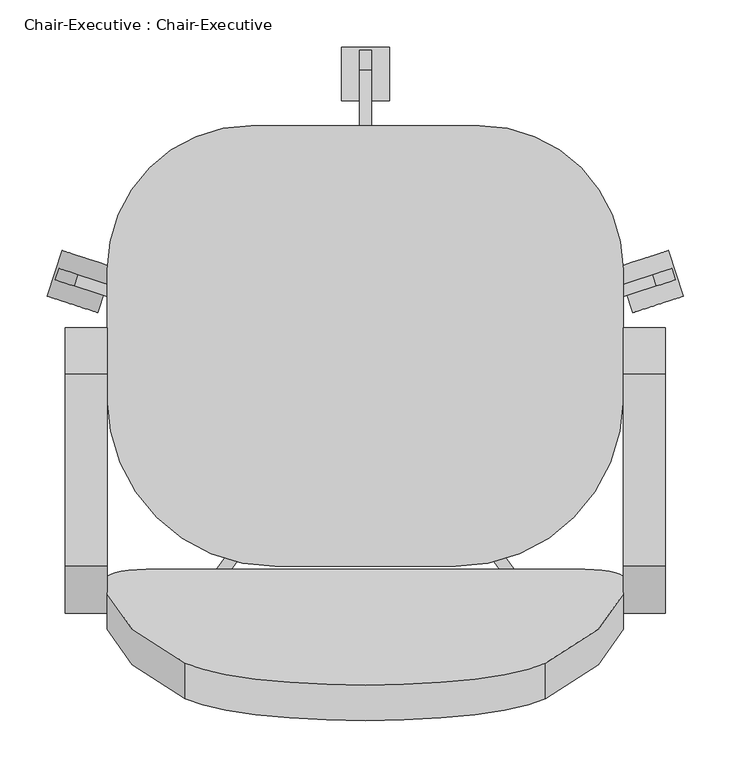
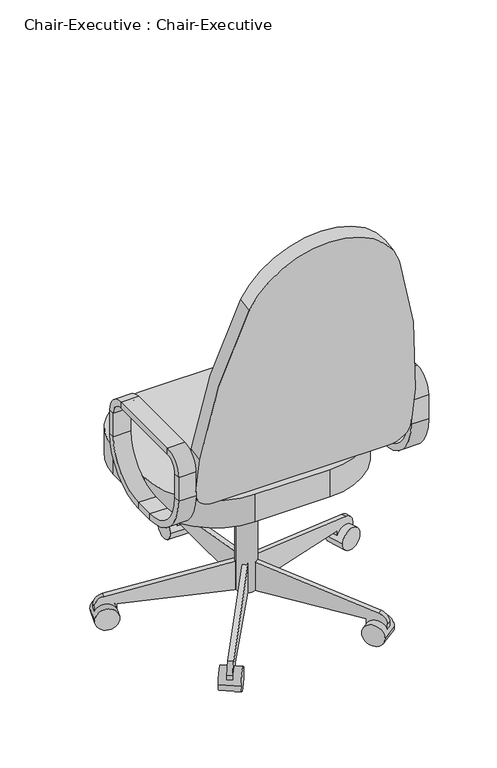
"""IFC4 building model written with IfcOpenShell, lengths in millimetres: furniture geometry, Chair-Executive : Chair-Executive."""

import ifcopenshell
import ifcopenshell.guid

model = None  # the IFC model being written
_history = None  # IfcOwnerHistory: only IFC2X3 demands one
_inside = {}  # id of a spatial element -> (the spatial element, [elements in it])
_under = {}  # id of a project, library or spatial element -> (it, [spatial elements below it])
_declared = {}  # id of a project -> (the project, [libraries it declares])
_typed = {}  # id of a type object -> (the type object, [elements of that type])
_made_of = {}  # id of a material, layer set ... -> (it, [elements and type objects made of it])


def new_model(schema):
    """Start an empty IFC model of exactly this schema.

    Asked for "IFC4X3", IfcOpenShell would pick the latest addendum, in which some entities
    have other attributes; the version numbers below select the first issue.
    IFC2X3 requires an IfcOwnerHistory on every rooted entity: one is made here for all.
    """
    global model, _history
    if schema == "IFC4X3":
        model = ifcopenshell.file(schema_version=(4, 3, 0, 0))
    else:
        model = ifcopenshell.file(schema=schema)
    _inside.clear()
    _under.clear()
    _declared.clear()
    _typed.clear()
    _made_of.clear()
    _history = None
    if model.schema == "IFC2X3":
        org = make("IfcOrganization", Name="unknown")
        user = make(
            "IfcPersonAndOrganization",
            ThePerson=make("IfcPerson", FamilyName="unknown"),
            TheOrganization=org,
        )
        app = make(
            "IfcApplication",
            ApplicationDeveloper=org,
            Version="unknown",
            ApplicationFullName="unknown",
            ApplicationIdentifier="unknown",
        )
        _history = make(
            "IfcOwnerHistory",
            OwningUser=user,
            OwningApplication=app,
            ChangeAction="ADDED",
            CreationDate=0,
        )
    return model


def make(cls, **values):
    """One entity of the class cls with the attributes given. An attribute that is None is left unset."""
    return model.create_entity(
        cls, **{name: value for name, value in values.items() if value is not None}
    )


def rooted(cls, **values):
    """An entity with a GlobalId (a new one), such as an element, a storey or a relation."""
    return make(cls, GlobalId=ifcopenshell.guid.new(), OwnerHistory=_history, **values)


def si_unit(unit_type, name, prefix=None):
    """IfcSIUnit, for example si_unit("LENGTHUNIT", "METRE", prefix="MILLI")."""
    return make("IfcSIUnit", UnitType=unit_type, Prefix=prefix, Name=name)


def assignment(units):
    """IfcUnitAssignment: the units of a project."""
    return None if units is None else make("IfcUnitAssignment", Units=units)


def point(xyz):
    """IfcCartesianPoint."""
    return None if xyz is None else make("IfcCartesianPoint", Coordinates=xyz)


def direction(xyz):
    """IfcDirection."""
    return None if xyz is None else make("IfcDirection", DirectionRatios=xyz)


def frame(location, z_axis=None, x_axis=None):
    """IfcAxis2Placement3D, a coordinate frame: its origin and axes. An axis left out is left unset."""
    return make(
        "IfcAxis2Placement3D",
        Location=point(location),
        Axis=direction(z_axis),
        RefDirection=direction(x_axis),
    )


def frame_2d(location, x_axis=None):
    """IfcAxis2Placement2D, a coordinate frame in the plane: its origin and x axis."""
    return make(
        "IfcAxis2Placement2D", Location=point(location), RefDirection=direction(x_axis)
    )


def origin():
    """The frame at (0, 0, 0) with its axes left unset."""
    return frame((0.0, 0.0, 0.0))


def place(relative_to, where):
    """IfcLocalPlacement: puts the frame where relative to a parent placement (None: the world)."""
    return make(
        "IfcLocalPlacement", PlacementRelTo=relative_to, RelativePlacement=where
    )


def context(
    kind, dimensions, precision=None, world=None, true_north=None, identifier=None
):
    """IfcGeometricRepresentationContext, for example the 3D "Model" context."""
    return make(
        "IfcGeometricRepresentationContext",
        ContextIdentifier=identifier,
        ContextType=kind,
        CoordinateSpaceDimension=dimensions,
        Precision=precision,
        WorldCoordinateSystem=world,
        TrueNorth=true_north,
    )


def project(units=None, contexts=None):
    """IfcProject with its units and contexts."""
    return rooted(
        "IfcProject",
        Name="project",
        RepresentationContexts=contexts,
        UnitsInContext=assignment(units),
    )


def spatial(cls, under=None, at=None, **own):
    """A site, building, storey or space (cls), placed at a placement, below another one or the project."""
    s = rooted(cls, ObjectPlacement=at, **own)
    if under is not None:
        _under.setdefault(under.id(), (under, []))[1].append(s)
    return s


def polyline(points):
    """IfcPolyline through the points."""
    return make("IfcPolyline", Points=[point(p) for p in points])


def circle_curve(where, radius):
    """IfcCircle in the frame where."""
    return make("IfcCircle", Position=where, Radius=radius)


def trimmed(basis, trim1, trim2, sense, master):
    """IfcTrimmedCurve: the piece of a basis curve between two trims."""
    return make(
        "IfcTrimmedCurve",
        BasisCurve=basis,
        Trim1=trim1,
        Trim2=trim2,
        SenseAgreement=sense,
        MasterRepresentation=master,
    )


def segment(curve, same_sense, transition):
    """IfcCompositeCurveSegment."""
    return make(
        "IfcCompositeCurveSegment",
        Transition=transition,
        SameSense=same_sense,
        ParentCurve=curve,
    )


def composite_curve(segments, self_intersect=None):
    """IfcCompositeCurve: segments joined end to end."""
    return make("IfcCompositeCurve", Segments=segments, SelfIntersect=self_intersect)


def outline(outer, holes=None, kind="AREA"):
    """IfcArbitraryClosedProfileDef: a profile drawn as a closed curve; with holes, ...WithVoids."""
    if holes is None:
        return make("IfcArbitraryClosedProfileDef", ProfileType=kind, OuterCurve=outer)
    return make(
        "IfcArbitraryProfileDefWithVoids",
        ProfileType=kind,
        OuterCurve=outer,
        InnerCurves=holes,
    )


def extrude(swept, where, along, depth):
    """IfcExtrudedAreaSolid: the profile swept, set in the frame where, extruded along a direction by depth."""
    return make(
        "IfcExtrudedAreaSolid",
        SweptArea=swept,
        Position=where,
        ExtrudedDirection=direction(along),
        Depth=depth,
    )


def shape(context_of_items, identifier, shape_type, items):
    """IfcShapeRepresentation: the items that make up one representation, for example the "Body"."""
    return make(
        "IfcShapeRepresentation",
        ContextOfItems=context_of_items,
        RepresentationIdentifier=identifier,
        RepresentationType=shape_type,
        Items=items,
    )


def source(mapping_origin, context_of_items, identifier, shape_type, items):
    """IfcRepresentationMap: a shape defined once, which mapped items show again and again."""
    return make(
        "IfcRepresentationMap",
        MappingOrigin=mapping_origin,
        MappedRepresentation=shape(context_of_items, identifier, shape_type, items),
    )


def transform(
    local_origin,
    x_axis=None,
    y_axis=None,
    z_axis=None,
    scale=None,
    scale2=None,
    scale3=None,
    uniform=True,
):
    """IfcCartesianTransformationOperator3D, or its non-uniform kind. x_axis, y_axis, z_axis: its Axis1, 2, 3."""
    if uniform:
        return make(
            "IfcCartesianTransformationOperator3D",
            Axis1=direction(x_axis),
            Axis2=direction(y_axis),
            LocalOrigin=point(local_origin),
            Scale=scale,
            Axis3=direction(z_axis),
        )
    return make(
        "IfcCartesianTransformationOperator3DnonUniform",
        Axis1=direction(x_axis),
        Axis2=direction(y_axis),
        LocalOrigin=point(local_origin),
        Scale=scale,
        Axis3=direction(z_axis),
        Scale2=scale2,
        Scale3=scale3,
    )


def mapped(mapping_source, mapping_target):
    """IfcMappedItem: shows the shape of a source again, moved by a transform."""
    return make(
        "IfcMappedItem", MappingSource=mapping_source, MappingTarget=mapping_target
    )


def made_of(thing, what):
    """Note that an element or type object is made of a material, layer set ...; save() writes the relation."""
    if what is not None:
        _made_of.setdefault(what.id(), (what, []))[1].append(thing)
    return thing


def element(
    cls,
    number,
    at=None,
    inside=None,
    cuts=None,
    type_object=None,
    material=None,
    context=None,
    identifier="Body",
    shape_type=None,
    held_by="IfcProductDefinitionShape",
    body=None,
    shapes=None,
    **own,
):
    """One element of the class cls, such as IfcWall. Its Tag is "e" and its number.

    at: its placement. inside: the storey or other place that contains it. cuts: it is an
    opening in that element (IfcRelVoidsElement). A single representation is given by context,
    identifier, shape_type and body (its items); several are given by shapes. held_by: the class
    of the entity that holds the representations. save() writes the other relations.
    """
    e = rooted(cls, Tag="e%d" % number, ObjectPlacement=at, **own)
    if body is not None:
        shapes = [shape(context, identifier, shape_type, body)]
    if shapes is not None:
        e.Representation = make(held_by, Representations=shapes)
    if inside is not None:
        _inside.setdefault(inside.id(), (inside, []))[1].append(e)
    if cuts is not None:
        rooted(
            "IfcRelVoidsElement", RelatingBuildingElement=cuts, RelatedOpeningElement=e
        )
    if type_object is not None:
        _typed.setdefault(type_object.id(), (type_object, []))[1].append(e)
    return made_of(e, material)


def aggregate(whole, parts):
    """IfcRelAggregates: a whole, such as a stair, and the parts it consists of."""
    return rooted("IfcRelAggregates", RelatingObject=whole, RelatedObjects=parts)


def save(model, path):
    """Write the relations noted so far, then the file.

    IfcRelAggregates (storeys below a building ...), IfcRelContainedInSpatialStructure (elements
    in a storey), IfcRelDefinesByType, IfcRelAssociatesMaterial and IfcRelDeclares: one each for
    every whole, place, type object, material and project.
    """
    for whole, parts in _under.values():
        aggregate(whole, parts)
    for where, things in _inside.values():
        rooted(
            "IfcRelContainedInSpatialStructure",
            RelatedElements=things,
            RelatingStructure=where,
        )
    for kind, things in _typed.values():
        rooted("IfcRelDefinesByType", RelatedObjects=things, RelatingType=kind)
    for what, things in _made_of.values():
        rooted("IfcRelAssociatesMaterial", RelatedObjects=things, RelatingMaterial=what)
    for by, libraries in _declared.values():
        rooted("IfcRelDeclares", RelatingContext=by, RelatedDefinitions=libraries)
    model.write(path)


def plane_surface(at):
    """IfcPlane: the flat surface through the origin of the frame at, square to its z axis."""
    return make("IfcPlane", Position=at)


def cylinder_surface(at, radius):
    """IfcCylindricalSurface: all points at the distance radius from the z axis of the frame at."""
    return make("IfcCylindricalSurface", Position=at, Radius=radius)


def revolved_surface(curve, axis_point, axis_direction):
    """IfcSurfaceOfRevolution: the curve turned about the line through axis_point along axis_direction."""
    return make(
        "IfcSurfaceOfRevolution",
        SweptCurve=make("IfcArbitraryOpenProfileDef", ProfileType="CURVE", Curve=curve),
        AxisPosition=make("IfcAxis1Placement", Location=point(axis_point), Axis=direction(axis_direction)),
    )


def advanced_brep(points, edges, surfaces, faces):
    """IfcAdvancedBrep: a solid bounded by faces that lie on surfaces and meet in shared edges.

    An edge is (start, end): straight between two places in points (the first is 0);
    or (start, end, curve); or (start, end, curve, False) where it runs against its curve.
    A face is (place in surfaces, loops), or (place, loops, False) where it looks against
    its surface's normal. A loop lists edges by number (the first is 1), with a minus sign
    where the edge is run from its end to its start. The first loop is the outer one.
    """
    corners = [point(p) for p in points]
    vertices = [make("IfcVertexPoint", VertexGeometry=c) for c in corners]
    made = []
    for start, end, *more in edges:
        made.append(
            make(
                "IfcEdgeCurve",
                EdgeStart=vertices[start],
                EdgeEnd=vertices[end],
                EdgeGeometry=more[0] if more else make("IfcPolyline", Points=[corners[start], corners[end]]),
                SameSense=more[1] if len(more) > 1 else True,
            )
        )
    hull = []
    for where, loops, *sense in faces:
        bounds = []
        for j, loop in enumerate(loops):
            ring = [make("IfcOrientedEdge", EdgeElement=made[abs(k) - 1], Orientation=k > 0) for k in loop]
            bounds.append(
                make(
                    "IfcFaceOuterBound" if j == 0 else "IfcFaceBound",
                    Bound=make("IfcEdgeLoop", EdgeList=ring),
                    Orientation=True,
                )
            )
        hull.append(make("IfcAdvancedFace", Bounds=bounds, FaceSurface=surfaces[where], SameSense=sense[0] if sense else True))
    return make("IfcAdvancedBrep", Outer=make("IfcClosedShell", CfsFaces=hull))


def chair_executive_chair_executive_8d69e98c(model_context):
    return source(origin(), model_context, "Body", "SolidModel", [
        advanced_brep(
        [(-176.5091803, -217.7873012, 546.1), (-176.5091803, -108.0540984, 436.3667972), (-176.5091803, -108.0540984, 420.4917972), (-176.5091803, -233.6623012, 546.1), (-132.0591803, -217.7873012, 546.1), (-132.0591803, -108.0540984, 436.3667972), (-132.0591803, -233.6623012, 546.1), (-132.0591803, -108.0540984, 420.4917972), (-176.5091803, -233.6623012, 609.6), (-176.5091803, -217.7873012, 609.6), (-132.0591803, -217.7873012, 609.6), (-132.0591803, -233.6623012, 609.6), (-176.5091803, -184.2540984, 643.1332028), (-176.5091803, -184.2540984, 659.0082028), (-132.0591803, -184.2540984, 643.1332028), (-132.0591803, -184.2540984, 659.0082028), (-176.5091803, 18.9459016, 659.0082028), (-176.5091803, 18.9459016, 643.1332028), (-132.0591803, 18.9459016, 643.1332028), (-132.0591803, 18.9459016, 659.0082028), (-176.5091803, 52.4791044, 609.6), (-176.5091803, 68.3541044, 609.6), (-132.0591803, 52.4791044, 609.6), (-132.0591803, 68.3541044, 609.6), (-176.5091803, 68.3541044, 546.1), (-176.5091803, 52.4791044, 546.1), (-132.0591803, 52.4791044, 546.1), (-132.0591803, 68.3541044, 546.1), (-176.5091803, -57.2540984, 436.3667972), (-176.5091803, -57.2540984, 420.4917972), (-132.0591803, -57.2540984, 436.3667972), (-132.0591803, -57.2540984, 420.4917972)],
        [
            (0, 1, circle_curve(frame((-176.5091803, -108.0540984, 546.1), z_axis=(1.0, 0.0, 0.0), x_axis=(0.0, 0.0, -1.0)), 109.7332028)),
            (1, 2),
            (2, 3, circle_curve(frame((-176.5091803, -108.0540984, 546.1), z_axis=(-1.0, 0.0, 0.0), x_axis=(0.0, 0.0, -1.0)), 125.6082028)),
            (3, 0),
            (4, 5, circle_curve(frame((-132.0591803, -108.0540984, 546.1), z_axis=(1.0, 0.0, 0.0), x_axis=(0.0, 0.0, -1.0)), 109.7332028)),
            (5, 1),
            (0, 4),
            (6, 7, circle_curve(frame((-132.0591803, -108.0540984, 546.1), z_axis=(1.0, 0.0, 0.0), x_axis=(0.0, 0.0, -1.0)), 125.6082028)),
            (7, 5),
            (4, 6),
            (2, 7),
            (6, 3),
            (3, 8),
            (8, 9),
            (9, 0),
            (9, 10),
            (10, 4),
            (10, 11),
            (11, 6),
            (11, 8),
            (12, 9, circle_curve(frame((-176.5091803, -184.2540984, 609.6), z_axis=(1.0, 0.0, 0.0), x_axis=(0.0, -1.0, 0.0)), 33.5332028)),
            (8, 13, circle_curve(frame((-176.5091803, -184.2540984, 609.6), z_axis=(-1.0, 0.0, 0.0), x_axis=(0.0, -1.0, 0.0)), 49.4082028)),
            (13, 12),
            (14, 10, circle_curve(frame((-132.0591803, -184.2540984, 609.6), z_axis=(1.0, 0.0, 0.0), x_axis=(0.0, -1.0, 0.0)), 33.5332028)),
            (12, 14),
            (15, 11, circle_curve(frame((-132.0591803, -184.2540984, 609.6), z_axis=(1.0, 0.0, 0.0), x_axis=(0.0, -1.0, 0.0)), 49.4082028)),
            (14, 15),
            (15, 13),
            (13, 16),
            (16, 17),
            (17, 12),
            (17, 18),
            (18, 14),
            (18, 19),
            (19, 15),
            (19, 16),
            (20, 17, circle_curve(frame((-176.5091803, 18.9459016, 609.6), z_axis=(1.0, 0.0, 0.0), x_axis=(0.0, 0.0, 1.0)), 33.5332028)),
            (16, 21, circle_curve(frame((-176.5091803, 18.9459016, 609.6), z_axis=(-1.0, 0.0, 0.0), x_axis=(0.0, 0.0, 1.0)), 49.4082028)),
            (21, 20),
            (22, 18, circle_curve(frame((-132.0591803, 18.9459016, 609.6), z_axis=(1.0, 0.0, 0.0), x_axis=(0.0, 0.0, 1.0)), 33.5332028)),
            (20, 22),
            (23, 19, circle_curve(frame((-132.0591803, 18.9459016, 609.6), z_axis=(1.0, 0.0, 0.0), x_axis=(0.0, 0.0, 1.0)), 49.4082028)),
            (22, 23),
            (23, 21),
            (21, 24),
            (24, 25),
            (25, 20),
            (25, 26),
            (26, 22),
            (26, 27),
            (27, 23),
            (27, 24),
            (28, 25, circle_curve(frame((-176.5091803, -57.2540984, 546.1), z_axis=(1.0, 0.0, 0.0), x_axis=(0.0, 1.0, 0.0)), 109.7332028)),
            (24, 29, circle_curve(frame((-176.5091803, -57.2540984, 546.1), z_axis=(-1.0, 0.0, 0.0), x_axis=(0.0, 1.0, 0.0)), 125.6082028)),
            (29, 28),
            (30, 26, circle_curve(frame((-132.0591803, -57.2540984, 546.1), z_axis=(1.0, 0.0, 0.0), x_axis=(0.0, 1.0, 0.0)), 109.7332028)),
            (28, 30),
            (31, 27, circle_curve(frame((-132.0591803, -57.2540984, 546.1), z_axis=(1.0, 0.0, 0.0), x_axis=(0.0, 1.0, 0.0)), 125.6082028)),
            (30, 31),
            (31, 29),
            (29, 2),
            (1, 28),
            (5, 30),
            (7, 31),
        ],
        [
            plane_surface(frame((-176.5091803, -108.0540984, 546.1), z_axis=(-1.0, 0.0, 0.0), x_axis=(0.0, 0.0, -1.0))),
            revolved_surface(polyline([(-176.5091803, -108.0540984, 436.3667972), (-132.0591803, -108.0540984, 436.3667972)]), (-132.0591803, -108.0540984, 546.1), (-1.0, 0.0, 0.0)),
            plane_surface(frame((-132.0591803, -108.0540984, 546.1), z_axis=(1.0, 0.0, 0.0), x_axis=(0.0, 0.0, -1.0))),
            cylinder_surface(frame((-132.0591803, -108.0540984, 546.1), z_axis=(-1.0, 0.0, 0.0), x_axis=(0.0, 0.0, -1.0)), 125.6082028),
            plane_surface(frame((-176.5091803, -233.6623012, 546.1), z_axis=(-1.0, 0.0, 0.0), x_axis=(0.0, 0.0, 1.0))),
            plane_surface(frame((-176.5091803, -217.7873012, 546.1), z_axis=(0.0, 1.0, 0.0), x_axis=(0.0, 0.0, 1.0))),
            plane_surface(frame((-132.0591803, -217.7873012, 546.1), z_axis=(1.0, 0.0, 0.0), x_axis=(0.0, 0.0, 1.0))),
            plane_surface(frame((-132.0591803, -233.6623012, 546.1), z_axis=(0.0, -1.0, 0.0), x_axis=(0.0, 0.0, 1.0))),
            plane_surface(frame((-176.5091803, -184.2540984, 609.6), z_axis=(-1.0, 0.0, 0.0), x_axis=(0.0, -1.0, 0.0))),
            revolved_surface(polyline([(-176.5091803, -217.7873012, 609.6), (-132.0591803, -217.7873012, 609.6)]), (-132.0591803, -184.2540984, 609.6), (-1.0, 0.0, 0.0)),
            plane_surface(frame((-132.0591803, -184.2540984, 609.6), z_axis=(1.0, 0.0, 0.0), x_axis=(0.0, -1.0, 0.0))),
            cylinder_surface(frame((-132.0591803, -184.2540984, 609.6), z_axis=(-1.0, 0.0, 0.0), x_axis=(0.0, -1.0, 0.0)), 49.4082028),
            plane_surface(frame((-176.5091803, -184.2540984, 659.0082028), z_axis=(-1.0, 0.0, 0.0), x_axis=(0.0, 1.0, 0.0))),
            plane_surface(frame((-176.5091803, -184.2540984, 643.1332028), z_axis=(0.0, 0.0, -1.0), x_axis=(0.0, 1.0, 0.0))),
            plane_surface(frame((-132.0591803, -184.2540984, 643.1332028), z_axis=(1.0, 0.0, 0.0), x_axis=(0.0, 1.0, 0.0))),
            plane_surface(frame((-132.0591803, -184.2540984, 659.0082028), z_axis=(0.0, 0.0, 1.0), x_axis=(0.0, 1.0, 0.0))),
            plane_surface(frame((-176.5091803, 18.9459016, 609.6), z_axis=(-1.0, 0.0, 0.0), x_axis=(0.0, 0.0, 1.0))),
            revolved_surface(polyline([(-176.5091803, 18.9459016, 643.1332028), (-132.0591803, 18.9459016, 643.1332028)]), (-132.0591803, 18.9459016, 609.6), (-1.0, 0.0, 0.0)),
            plane_surface(frame((-132.0591803, 18.9459016, 609.6), z_axis=(1.0, 0.0, 0.0), x_axis=(0.0, 0.0, 1.0))),
            cylinder_surface(frame((-132.0591803, 18.9459016, 609.6), z_axis=(-1.0, 0.0, 0.0), x_axis=(0.0, 0.0, 1.0)), 49.4082028),
            plane_surface(frame((-176.5091803, 68.3541044, 609.6), z_axis=(-1.0, 0.0, 0.0), x_axis=(0.0, 0.0, -1.0))),
            plane_surface(frame((-176.5091803, 52.4791044, 609.6), z_axis=(0.0, -1.0, 0.0), x_axis=(0.0, 0.0, -1.0))),
            plane_surface(frame((-132.0591803, 52.4791044, 609.6), z_axis=(1.0, 0.0, 0.0), x_axis=(0.0, 0.0, -1.0))),
            plane_surface(frame((-132.0591803, 68.3541044, 609.6), z_axis=(0.0, 1.0, 0.0), x_axis=(0.0, 0.0, -1.0))),
            plane_surface(frame((-176.5091803, -57.2540984, 546.1), z_axis=(-1.0, 0.0, 0.0), x_axis=(0.0, 1.0, 0.0))),
            revolved_surface(polyline([(-176.5091803, 52.479104400000004, 546.1), (-132.0591803, 52.479104400000004, 546.1)]), (-132.0591803, -57.2540984, 546.1), (-1.0, 0.0, 0.0)),
            plane_surface(frame((-132.0591803, -57.2540984, 546.1), z_axis=(1.0, 0.0, 0.0), x_axis=(0.0, 1.0, 0.0))),
            cylinder_surface(frame((-132.0591803, -57.2540984, 546.1), z_axis=(-1.0, 0.0, 0.0), x_axis=(0.0, 1.0, 0.0)), 125.6082028),
            plane_surface(frame((-176.5091803, -57.2540984, 420.4917972), z_axis=(-1.0, 0.0, 0.0), x_axis=(0.0, -1.0, 0.0))),
            plane_surface(frame((-176.5091803, -57.2540984, 436.3667972), z_axis=(0.0, 0.0, 1.0), x_axis=(0.0, -1.0, 0.0))),
            plane_surface(frame((-132.0591803, -57.2540984, 436.3667972), z_axis=(1.0, 0.0, 0.0), x_axis=(0.0, -1.0, 0.0))),
            plane_surface(frame((-132.0591803, -57.2540984, 420.4917972), z_axis=(0.0, 0.0, -1.0), x_axis=(0.0, -1.0, 0.0))),
        ],
        [
            (0, [[1, 2, 3, 4]]),
            (1, [[5, 6, -1, 7]]),
            (2, [[8, 9, -5, 10]]),
            (3, [[-3, 11, -8, 12]]),
            (4, [[-4, 13, 14, 15]]),
            (5, [[-7, -15, 16, 17]]),
            (6, [[-10, -17, 18, 19]]),
            (7, [[-12, -19, 20, -13]]),
            (8, [[21, -14, 22, 23]]),
            (9, [[24, -16, -21, 25]]),
            (10, [[26, -18, -24, 27]]),
            (11, [[-22, -20, -26, 28]]),
            (12, [[-23, 29, 30, 31]]),
            (13, [[-25, -31, 32, 33]]),
            (14, [[-27, -33, 34, 35]]),
            (15, [[-28, -35, 36, -29]]),
            (16, [[37, -30, 38, 39]]),
            (17, [[40, -32, -37, 41]]),
            (18, [[42, -34, -40, 43]]),
            (19, [[-38, -36, -42, 44]]),
            (20, [[-39, 45, 46, 47]]),
            (21, [[-41, -47, 48, 49]]),
            (22, [[-43, -49, 50, 51]]),
            (23, [[-44, -51, 52, -45]]),
            (24, [[53, -46, 54, 55]]),
            (25, [[56, -48, -53, 57]]),
            (26, [[58, -50, -56, 59]]),
            (27, [[-54, -52, -58, 60]]),
            (28, [[-55, 61, -2, 62]]),
            (29, [[-57, -62, -6, 63]]),
            (30, [[-59, -63, -9, 64]]),
            (31, [[-60, -64, -11, -61]]),
        ],
    ),
        advanced_brep(
        [(414.0408197, -233.6623012, 546.1), (414.0408197, -108.0540984, 420.4917972), (458.4908197, -108.0540984, 420.4917972), (458.4908197, -233.6623012, 546.1), (414.0408197, -217.7873012, 546.1), (414.0408197, -108.0540984, 436.3667972), (458.4908197, -217.7873012, 546.1), (458.4908197, -108.0540984, 436.3667972), (458.4908197, -233.6623012, 609.6), (414.0408197, -233.6623012, 609.6), (414.0408197, -217.7873012, 609.6), (458.4908197, -217.7873012, 609.6), (414.0408197, -184.2540984, 659.0082028), (458.4908197, -184.2540984, 659.0082028), (414.0408197, -184.2540984, 643.1332028), (458.4908197, -184.2540984, 643.1332028), (458.4908197, 18.9459016, 659.0082028), (414.0408197, 18.9459016, 659.0082028), (414.0408197, 18.9459016, 643.1332028), (458.4908197, 18.9459016, 643.1332028), (414.0408197, 68.3541044, 609.6), (458.4908197, 68.3541044, 609.6), (414.0408197, 52.4791044, 609.6), (458.4908197, 52.4791044, 609.6), (458.4908197, 68.3541044, 546.1), (414.0408197, 68.3541044, 546.1), (414.0408197, 52.4791044, 546.1), (458.4908197, 52.4791044, 546.1), (414.0408197, -57.2540984, 420.4917972), (458.4908197, -57.2540984, 420.4917972), (414.0408197, -57.2540984, 436.3667972), (458.4908197, -57.2540984, 436.3667972)],
        [
            (0, 1, circle_curve(frame((414.0408197, -108.0540984, 546.1), z_axis=(1.0, 0.0, 0.0), x_axis=(0.0, 0.0, -1.0)), 125.6082028)),
            (1, 2),
            (2, 3, circle_curve(frame((458.4908197, -108.0540984, 546.1), z_axis=(-1.0, 0.0, 0.0), x_axis=(0.0, 0.0, -1.0)), 125.6082028)),
            (3, 0),
            (4, 5, circle_curve(frame((414.0408197, -108.0540984, 546.1), z_axis=(1.0, 0.0, 0.0), x_axis=(0.0, 0.0, -1.0)), 109.7332028)),
            (5, 1),
            (0, 4),
            (6, 7, circle_curve(frame((458.4908197, -108.0540984, 546.1), z_axis=(1.0, 0.0, 0.0), x_axis=(0.0, 0.0, -1.0)), 109.7332028)),
            (7, 5),
            (4, 6),
            (2, 7),
            (6, 3),
            (3, 8),
            (8, 9),
            (9, 0),
            (9, 10),
            (10, 4),
            (10, 11),
            (11, 6),
            (11, 8),
            (12, 9, circle_curve(frame((414.0408197, -184.2540984, 609.6), z_axis=(1.0, 0.0, 0.0), x_axis=(0.0, -1.0, 0.0)), 49.4082028)),
            (8, 13, circle_curve(frame((458.4908197, -184.2540984, 609.6), z_axis=(-1.0, 0.0, 0.0), x_axis=(0.0, -1.0, 0.0)), 49.4082028)),
            (13, 12),
            (14, 10, circle_curve(frame((414.0408197, -184.2540984, 609.6), z_axis=(1.0, 0.0, 0.0), x_axis=(0.0, -1.0, 0.0)), 33.5332028)),
            (12, 14),
            (15, 11, circle_curve(frame((458.4908197, -184.2540984, 609.6), z_axis=(1.0, 0.0, 0.0), x_axis=(0.0, -1.0, 0.0)), 33.5332028)),
            (14, 15),
            (15, 13),
            (13, 16),
            (16, 17),
            (17, 12),
            (17, 18),
            (18, 14),
            (18, 19),
            (19, 15),
            (19, 16),
            (20, 17, circle_curve(frame((414.0408197, 18.9459016, 609.6), z_axis=(1.0, 0.0, 0.0), x_axis=(0.0, 0.0, 1.0)), 49.4082028)),
            (16, 21, circle_curve(frame((458.4908197, 18.9459016, 609.6), z_axis=(-1.0, 0.0, 0.0), x_axis=(0.0, 0.0, 1.0)), 49.4082028)),
            (21, 20),
            (22, 18, circle_curve(frame((414.0408197, 18.9459016, 609.6), z_axis=(1.0, 0.0, 0.0), x_axis=(0.0, 0.0, 1.0)), 33.5332028)),
            (20, 22),
            (23, 19, circle_curve(frame((458.4908197, 18.9459016, 609.6), z_axis=(1.0, 0.0, 0.0), x_axis=(0.0, 0.0, 1.0)), 33.5332028)),
            (22, 23),
            (23, 21),
            (21, 24),
            (24, 25),
            (25, 20),
            (25, 26),
            (26, 22),
            (26, 27),
            (27, 23),
            (27, 24),
            (28, 25, circle_curve(frame((414.0408197, -57.2540984, 546.1), z_axis=(1.0, 0.0, 0.0), x_axis=(0.0, 1.0, 0.0)), 125.6082028)),
            (24, 29, circle_curve(frame((458.4908197, -57.2540984, 546.1), z_axis=(-1.0, 0.0, 0.0), x_axis=(0.0, 1.0, 0.0)), 125.6082028)),
            (29, 28),
            (30, 26, circle_curve(frame((414.0408197, -57.2540984, 546.1), z_axis=(1.0, 0.0, 0.0), x_axis=(0.0, 1.0, 0.0)), 109.7332028)),
            (28, 30),
            (31, 27, circle_curve(frame((458.4908197, -57.2540984, 546.1), z_axis=(1.0, 0.0, 0.0), x_axis=(0.0, 1.0, 0.0)), 109.7332028)),
            (30, 31),
            (31, 29),
            (29, 2),
            (1, 28),
            (5, 30),
            (7, 31),
        ],
        [
            cylinder_surface(frame((414.0408197, -108.0540984, 546.1), z_axis=(-1.0, 0.0, 0.0), x_axis=(0.0, 0.0, -1.0)), 125.6082028),
            plane_surface(frame((414.0408197, -108.0540984, 546.1), z_axis=(-1.0, 0.0, 0.0), x_axis=(0.0, 0.0, -1.0))),
            revolved_surface(polyline([(414.0408197, -108.0540984, 436.3667972), (458.4908197, -108.0540984, 436.3667972)]), (414.0408197, -108.0540984, 546.1), (-1.0, 0.0, 0.0)),
            plane_surface(frame((458.4908197, -108.0540984, 546.1), z_axis=(1.0, 0.0, 0.0), x_axis=(0.0, 0.0, -1.0))),
            plane_surface(frame((458.4908197, -233.6623012, 546.1), z_axis=(0.0, -1.0, 0.0), x_axis=(0.0, 0.0, 1.0))),
            plane_surface(frame((414.0408197, -233.6623012, 546.1), z_axis=(-1.0, 0.0, 0.0), x_axis=(0.0, 0.0, 1.0))),
            plane_surface(frame((414.0408197, -217.7873012, 546.1), z_axis=(0.0, 1.0, 0.0), x_axis=(0.0, 0.0, 1.0))),
            plane_surface(frame((458.4908197, -217.7873012, 546.1), z_axis=(1.0, 0.0, 0.0), x_axis=(0.0, 0.0, 1.0))),
            cylinder_surface(frame((414.0408197, -184.2540984, 609.6), z_axis=(-1.0, 0.0, 0.0), x_axis=(0.0, -1.0, 0.0)), 49.4082028),
            plane_surface(frame((414.0408197, -184.2540984, 609.6), z_axis=(-1.0, 0.0, 0.0), x_axis=(0.0, -1.0, 0.0))),
            revolved_surface(polyline([(414.0408197, -217.7873012, 609.6), (458.4908197, -217.7873012, 609.6)]), (414.0408197, -184.2540984, 609.6), (-1.0, 0.0, 0.0)),
            plane_surface(frame((458.4908197, -184.2540984, 609.6), z_axis=(1.0, 0.0, 0.0), x_axis=(0.0, -1.0, 0.0))),
            plane_surface(frame((458.4908197, -184.2540984, 659.0082028), z_axis=(0.0, 0.0, 1.0), x_axis=(0.0, 1.0, 0.0))),
            plane_surface(frame((414.0408197, -184.2540984, 659.0082028), z_axis=(-1.0, 0.0, 0.0), x_axis=(0.0, 1.0, 0.0))),
            plane_surface(frame((414.0408197, -184.2540984, 643.1332028), z_axis=(0.0, 0.0, -1.0), x_axis=(0.0, 1.0, 0.0))),
            plane_surface(frame((458.4908197, -184.2540984, 643.1332028), z_axis=(1.0, 0.0, 0.0), x_axis=(0.0, 1.0, 0.0))),
            cylinder_surface(frame((414.0408197, 18.9459016, 609.6), z_axis=(-1.0, 0.0, 0.0), x_axis=(0.0, 0.0, 1.0)), 49.4082028),
            plane_surface(frame((414.0408197, 18.9459016, 609.6), z_axis=(-1.0, 0.0, 0.0), x_axis=(0.0, 0.0, 1.0))),
            revolved_surface(polyline([(414.0408197, 18.9459016, 643.1332028), (458.4908197, 18.9459016, 643.1332028)]), (414.0408197, 18.9459016, 609.6), (-1.0, 0.0, 0.0)),
            plane_surface(frame((458.4908197, 18.9459016, 609.6), z_axis=(1.0, 0.0, 0.0), x_axis=(0.0, 0.0, 1.0))),
            plane_surface(frame((458.4908197, 68.3541044, 609.6), z_axis=(0.0, 1.0, 0.0), x_axis=(0.0, 0.0, -1.0))),
            plane_surface(frame((414.0408197, 68.3541044, 609.6), z_axis=(-1.0, 0.0, 0.0), x_axis=(0.0, 0.0, -1.0))),
            plane_surface(frame((414.0408197, 52.4791044, 609.6), z_axis=(0.0, -1.0, 0.0), x_axis=(0.0, 0.0, -1.0))),
            plane_surface(frame((458.4908197, 52.4791044, 609.6), z_axis=(1.0, 0.0, 0.0), x_axis=(0.0, 0.0, -1.0))),
            cylinder_surface(frame((414.0408197, -57.2540984, 546.1), z_axis=(-1.0, 0.0, 0.0), x_axis=(0.0, 1.0, 0.0)), 125.6082028),
            plane_surface(frame((414.0408197, -57.2540984, 546.1), z_axis=(-1.0, 0.0, 0.0), x_axis=(0.0, 1.0, 0.0))),
            revolved_surface(polyline([(414.0408197, 52.479104400000004, 546.1), (458.4908197, 52.479104400000004, 546.1)]), (414.0408197, -57.2540984, 546.1), (-1.0, 0.0, 0.0)),
            plane_surface(frame((458.4908197, -57.2540984, 546.1), z_axis=(1.0, 0.0, 0.0), x_axis=(0.0, 1.0, 0.0))),
            plane_surface(frame((458.4908197, -57.2540984, 420.4917972), z_axis=(0.0, 0.0, -1.0), x_axis=(0.0, -1.0, 0.0))),
            plane_surface(frame((414.0408197, -57.2540984, 420.4917972), z_axis=(-1.0, 0.0, 0.0), x_axis=(0.0, -1.0, 0.0))),
            plane_surface(frame((414.0408197, -57.2540984, 436.3667972), z_axis=(0.0, 0.0, 1.0), x_axis=(0.0, -1.0, 0.0))),
            plane_surface(frame((458.4908197, -57.2540984, 436.3667972), z_axis=(1.0, 0.0, 0.0), x_axis=(0.0, -1.0, 0.0))),
        ],
        [
            (0, [[1, 2, 3, 4]]),
            (1, [[5, 6, -1, 7]]),
            (2, [[8, 9, -5, 10]]),
            (3, [[-3, 11, -8, 12]]),
            (4, [[-4, 13, 14, 15]]),
            (5, [[-7, -15, 16, 17]]),
            (6, [[-10, -17, 18, 19]]),
            (7, [[-12, -19, 20, -13]]),
            (8, [[21, -14, 22, 23]]),
            (9, [[24, -16, -21, 25]]),
            (10, [[26, -18, -24, 27]]),
            (11, [[-22, -20, -26, 28]]),
            (12, [[-23, 29, 30, 31]]),
            (13, [[-25, -31, 32, 33]]),
            (14, [[-27, -33, 34, 35]]),
            (15, [[-28, -35, 36, -29]]),
            (16, [[37, -30, 38, 39]]),
            (17, [[40, -32, -37, 41]]),
            (18, [[42, -34, -40, 43]]),
            (19, [[-38, -36, -42, 44]]),
            (20, [[-39, 45, 46, 47]]),
            (21, [[-41, -47, 48, 49]]),
            (22, [[-43, -49, 50, 51]]),
            (23, [[-44, -51, 52, -45]]),
            (24, [[53, -46, 54, 55]]),
            (25, [[56, -48, -53, 57]]),
            (26, [[58, -50, -56, 59]]),
            (27, [[-54, -52, -58, 60]]),
            (28, [[-55, 61, -2, 62]]),
            (29, [[-57, -62, -6, 63]]),
            (30, [[-59, -63, -9, 64]]),
            (31, [[-60, -64, -11, -61]]),
        ],
    ),
        extrude(outline(composite_curve([segment(trimmed(circle_curve(frame_2d((0.0, -50.8)), 50.8), [point((0.0, 0.0))], [point((50.8, -50.8))], False, "CARTESIAN"), True, "CONTINUOUS"), segment(polyline([(50.8, -50.8), (50.8, -152.4)]), True, "CONTINUOUS"), segment(trimmed(circle_curve(frame_2d((-1471.2021854, -74.3913617)), 1524.0), [point((50.8, -152.4))], [point((-31.75, -574.9444618))], False, "CARTESIAN"), True, "CONTINUOUS"), segment(trimmed(circle_curve(frame_2d((-222.25, -504.2338544)), 203.2), [point((-31.75, -574.9444618))], [point((-412.75, -574.9444618))], False, "CARTESIAN"), True, "CONTINUOUS"), segment(trimmed(circle_curve(frame_2d((1026.7021854, -74.3913617)), 1524.0), [point((-412.75, -574.9444618))], [point((-495.3, -152.4))], False, "CARTESIAN"), True, "CONTINUOUS"), segment(polyline([(-495.3, -152.4), (-495.3, -50.8)]), True, "CONTINUOUS"), segment(trimmed(circle_curve(frame_2d((-444.5, -50.8)), 50.8), [point((-495.3, -50.8))], [point((-444.5, 0.0))], False, "CARTESIAN"), True, "CONTINUOUS"), segment(polyline([(-444.5, 0.0), (0.0, 0.0)]), True, "CONTINUOUS")], self_intersect=False)), frame((363.2408197, -224.5698964, 503.1641822), z_axis=(0.0, 0.9848077530122084, 0.17364817766692853), x_axis=(1.0, 0.0, 0.0)), (0.0, 0.0, 1.0), 38.1),
        extrude(outline(composite_curve([segment(trimmed(circle_curve(frame_2d((20.3408197, 129.4961016)), 152.4), [point((-132.0591803, 129.4961016))], [point((20.3408197, 281.8961016))], False, "CARTESIAN"), True, "CONTINUOUS"), segment(polyline([(20.3408197, 281.8961016), (261.6408197, 281.8961016)]), True, "CONTINUOUS"), segment(trimmed(circle_curve(frame_2d((261.6408197, 129.4961016)), 152.4), [point((261.6408197, 281.8961016))], [point((414.0408197, 129.4961016))], False, "CARTESIAN"), True, "CONTINUOUS"), segment(polyline([(414.0408197, 129.4961016), (414.0408197, -6.4540984)]), True, "CONTINUOUS"), segment(trimmed(circle_curve(frame_2d((236.2408197, -6.4540984)), 177.8), [point((414.0408197, -6.4540984))], [point((236.2408197, -184.2540984))], False, "CARTESIAN"), True, "CONTINUOUS"), segment(polyline([(236.2408197, -184.2540984), (45.7408197, -184.2540984)]), True, "CONTINUOUS"), segment(trimmed(circle_curve(frame_2d((45.7408197, -6.4540984)), 177.8), [point((45.7408197, -184.2540984))], [point((-132.0591803, -6.4540984))], False, "CARTESIAN"), True, "CONTINUOUS"), segment(polyline([(-132.0591803, -6.4540984), (-132.0591803, 129.4961016)]), True, "CONTINUOUS")], self_intersect=False)), frame((0.0, 0.0, 383.7835944), z_axis=(0.0, 0.0, 1.0), x_axis=(1.0, 0.0, 0.0)), (0.0, 0.0, 1.0), 73.4164056),
        extrude(outline(composite_curve([segment(trimmed(circle_curve(frame_2d((140.9908197, 18.9459016)), 25.4), [point((115.5908197, 18.9459016))], [point((166.3908197, 18.9459016))], False, "CARTESIAN"), True, "CONTINUOUS"), segment(trimmed(circle_curve(frame_2d((140.9908197, 18.9459016)), 25.4), [point((166.3908197, 18.9459016))], [point((115.5908197, 18.9459016))], False, "CARTESIAN"), True, "CONTINUOUS")], self_intersect=False)), frame((0.0, 0.0, 53.5835944), z_axis=(0.0, 0.0, 1.0), x_axis=(1.0, 0.0, 0.0)), (0.0, 0.0, 1.0), 330.5914056),
        extrude(outline(composite_curve([segment(trimmed(circle_curve(frame_2d((0.0, -28.2002727)), 28.2002727), [point((0.0, -56.4005455))], [point((0.0, 0.0))], False, "CARTESIAN"), True, "CONTINUOUS"), segment(trimmed(circle_curve(frame_2d((0.0, -28.2002727)), 28.2002727), [point((0.0, 0.0))], [point((0.0, -56.4005455))], False, "CARTESIAN"), True, "CONTINUOUS")], self_intersect=False)), frame((477.6203484, 101.6163254, 28.1835944), z_axis=(-0.3090169943749423, 0.9510565162951553, 0.0), x_axis=(0.0, 0.0, 1.0)), (0.0, 0.0, 1.0), 50.8),
        extrude(outline(composite_curve([segment(polyline([(-25.4, 0.0), (0.0, 0.0), (0.0, -50.8), (-24.303053, -50.8)]), True, "CONTINUOUS"), segment(trimmed(circle_curve(frame_2d((-24.303053, -25.4)), 25.4), [point((-24.303053, -50.8))], [point((-49.3171699, -29.8106637))], False, "CARTESIAN"), True, "CONTINUOUS"), segment(polyline([(-49.3171699, -29.8106637), (-101.6, 266.7), (-101.6, 292.1), (-25.4, 292.1), (-25.4, 0.0)]), True, "CONTINUOUS")], self_intersect=False)), frame((420.756686, 103.1705568, 28.1835944), z_axis=(-0.3090169943749423, 0.9510565162951553, 0.0), x_axis=(0.0, 0.0, -1.0)), (0.0, 0.0, 1.0), 12.7),
        extrude(outline(composite_curve([segment(trimmed(circle_curve(frame_2d((0.0, -28.2002727)), 28.2002727), [point((0.0, -56.4005455))], [point((0.0, 0.0))], False, "CARTESIAN"), True, "CONTINUOUS"), segment(trimmed(circle_curve(frame_2d((0.0, -28.2002727)), 28.2002727), [point((0.0, 0.0))], [point((0.0, -56.4005455))], False, "CARTESIAN"), True, "CONTINUOUS")], self_intersect=False)), frame((323.63931, -275.6612394, 28.1835944), z_axis=(0.8090169943749499, 0.5877852522924699, 0.0), x_axis=(0.0, 0.0, 1.0)), (0.0, 0.0, 1.0), 50.8),
        extrude(outline(composite_curve([segment(polyline([(-25.4, 0.0), (0.0, 0.0), (0.0, -50.8), (-24.303053, -50.8)]), True, "CONTINUOUS"), segment(trimmed(circle_curve(frame_2d((-24.303053, -25.3999999)), 25.4), [point((-24.303053, -50.8))], [point((-49.3171699, -29.8106636))], False, "CARTESIAN"), True, "CONTINUOUS"), segment(polyline([(-49.3171699, -29.8106636), (-101.6, 266.7), (-101.6, 292.1), (-25.4, 292.1), (-25.4, 0.0)]), True, "CONTINUOUS")], self_intersect=False)), frame((307.545634, -221.1003988, 28.1835944), z_axis=(0.8090169943749499, 0.5877852522924699, 0.0), x_axis=(0.0, 0.0, -1.0)), (0.0, 0.0, 1.0), 12.7),
        extrude(outline(composite_curve([segment(trimmed(circle_curve(frame_2d((0.0, -28.2002727)), 28.2002727), [point((0.0, -56.4005455))], [point((0.0, 0.0))], False, "CARTESIAN"), True, "CONTINUOUS"), segment(trimmed(circle_curve(frame_2d((0.0, -28.2002727)), 28.2002727), [point((0.0, 0.0))], [point((0.0, -56.4005455))], False, "CARTESIAN"), True, "CONTINUOUS")], self_intersect=False)), frame((-41.6576707, -275.6612394, 28.1835944), z_axis=(-0.8090169943749458, 0.5877852522924754, 0.0), x_axis=(0.0, 0.0, -1.0)), (0.0, 0.0, 1.0), 50.8),
        extrude(outline(composite_curve([segment(polyline([(25.4, 0.0), (25.4, 292.1), (101.6, 292.1), (101.6, 266.7), (49.3171699, -29.8106637)]), True, "CONTINUOUS"), segment(trimmed(circle_curve(frame_2d((24.303053, -25.3999999)), 25.4), [point((49.3171699, -29.8106637))], [point((24.303053, -50.8))], False, "CARTESIAN"), True, "CONTINUOUS"), segment(polyline([(24.303053, -50.8), (0.0, -50.8), (0.0, 0.0), (25.4, 0.0)]), True, "CONTINUOUS")], self_intersect=False)), frame((-25.5639946, -221.1003988, 28.1835944), z_axis=(-0.8090169943749459, 0.5877852522924754, 0.0), x_axis=(0.0, 0.0, 1.0)), (0.0, 0.0, 1.0), 12.7),
        extrude(outline(composite_curve([segment(trimmed(circle_curve(frame_2d((0.0, -28.2002727)), 28.2002727), [point((0.0, -56.4005454))], [point((0.0, 0.0))], False, "CARTESIAN"), True, "CONTINUOUS"), segment(trimmed(circle_curve(frame_2d((0.0, -28.2002727)), 28.2002727), [point((0.0, 0.0))], [point((0.0, -56.4005454))], False, "CARTESIAN"), True, "CONTINUOUS")], self_intersect=False)), frame((-195.638709, 101.6163254, 28.1835944), z_axis=(0.3090169943749487, 0.9510565162951532, 0.0), x_axis=(0.0, 0.0, -1.0)), (0.0, 0.0, 1.0), 50.8),
        extrude(outline(composite_curve([segment(polyline([(25.4, 0.0), (25.4, 292.1000001), (101.6, 292.1000001), (101.6, 266.7), (49.3171699, -29.8106636)]), True, "CONTINUOUS"), segment(trimmed(circle_curve(frame_2d((24.303053, -25.4)), 25.4), [point((49.3171699, -29.8106636))], [point((24.303053, -50.8))], False, "CARTESIAN"), True, "CONTINUOUS"), segment(polyline([(24.303053, -50.8), (0.0, -50.8), (0.0, 0.0), (25.4, 0.0)]), True, "CONTINUOUS")], self_intersect=False)), frame((-138.7750467, 103.1705568, 28.1835944), z_axis=(0.3090169943749487, 0.9510565162951532, 0.0), x_axis=(0.0, 0.0, 1.0)), (0.0, 0.0, 1.0), 12.7),
        extrude(outline(composite_curve([segment(trimmed(circle_curve(frame_2d((336.4459016, 28.1835944)), 28.2002727), [point((308.2456289, 28.1835944))], [point((364.6461744, 28.1835944))], False, "CARTESIAN"), True, "CONTINUOUS"), segment(trimmed(circle_curve(frame_2d((336.4459016, 28.1835944)), 28.2002727), [point((364.6461744, 28.1835944))], [point((308.2456289, 28.1835944))], False, "CARTESIAN"), True, "CONTINUOUS")], self_intersect=False)), frame((115.5908197, 0.0, 0.0), z_axis=(1.0, 0.0, 0.0), x_axis=(0.0, 1.0, 0.0)), (0.0, 0.0, 1.0), 50.8),
        extrude(outline(composite_curve([segment(polyline([(311.0459016, 53.5835944), (18.9459016, 53.5835944), (18.9459016, 129.7835944), (44.3459016, 129.7835944), (340.8565654, 77.5007643)]), True, "CONTINUOUS"), segment(trimmed(circle_curve(frame_2d((336.4459016, 52.4866474)), 25.4), [point((340.8565654, 77.5007643))], [point((361.8459016, 52.4866474))], False, "CARTESIAN"), True, "CONTINUOUS"), segment(polyline([(361.8459016, 52.4866474), (361.8459016, 28.1835944), (311.0459016, 28.1835944), (311.0459016, 53.5835944)]), True, "CONTINUOUS")], self_intersect=False)), frame((134.6408197, 0.0, 0.0), z_axis=(1.0, 0.0, 0.0), x_axis=(0.0, 1.0, 0.0)), (0.0, 0.0, 1.0), 12.7),
        extrude(outline(polyline([(69.7459016, 383.7835944), (69.7459016, 371.0835944), (18.9459016, 283.0954134), (-19.1540984, 283.0954134), (-19.1540984, 383.7835944), (69.7459016, 383.7835944)])), frame((90.1908197, 0.0, 0.0), z_axis=(1.0, 0.0, 0.0), x_axis=(0.0, 1.0, 0.0)), (0.0, 0.0, 1.0), 101.6),
    ])


if __name__ == "__main__":
    model = new_model("IFC4")
    model_context = context("Model", 3, world=origin())
    ifc_project = project(units=[si_unit("LENGTHUNIT", "METRE", prefix="MILLI")], contexts=[model_context])
    site = spatial("IfcSite", under=ifc_project)
    building = spatial("IfcBuilding", under=site)
    placement = place(None, origin())
    chair_executive_chair_executive_shape = chair_executive_chair_executive_8d69e98c(model_context)
    element("IfcFurniture", 1, ObjectType="Chair-Executive : Chair-Executive", at=placement, inside=building, context=model_context, shape_type="MappedRepresentation", body=[
        mapped(chair_executive_chair_executive_shape, transform((0.0, 0.0, 0.0), x_axis=(1.0, 0.0, 0.0), y_axis=(0.0, 1.0, 0.0), z_axis=(0.0, 0.0, 1.0))),
    ])
    save(model, "model.ifc")

# Revit data of these elements
# Type "Chair-Executive : Chair-Executive"
#   Model = "ExecuChair"
#   Manufacturer = "Acme Furniture"
#   Type Mark = "CH-1"
#   Model = "ExecuChair"
#   Manufacturer = "Acme Furniture"
#   Assembly Code = "E2020200"
#   Cost = 875
#   Cost = 875
#   Type Image = Task Chair.png
#   Base/Arms Material = Plastic, Opaque Black
#   Casters Material = Plastic, Opaque Black
#   Seat/Back Material = Textile - Slate Blue
#   Default Elevation = 0
# Element 1 (IfcFurniture, "Chair-Executive : Chair-Executive")
#   Materials on its faces: "Plastic, Opaque Black", "Textile - Slate Blue"
# Materials
#   "Plastic, Opaque Black": class "Plastic", colour RGB 0 0 0, transparency 0, Description = "Plastic, generic, opaque black", Cost = 0
#   "Textile - Slate Blue": class "Fabric", colour RGB 98 102 118, transparency 0
